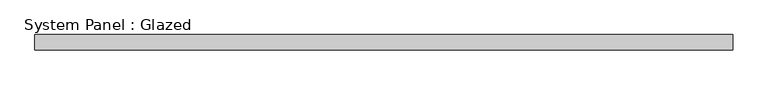
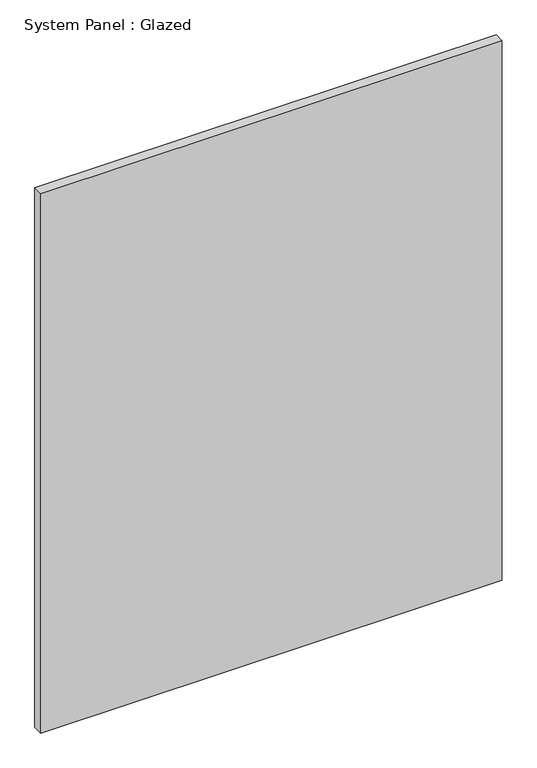
"""IFC4 building model written with IfcOpenShell, lengths in millimetres: plate geometry, System Panel : Glazed."""

import ifcopenshell
import ifcopenshell.guid

model = None  # the IFC model being written
_history = None  # IfcOwnerHistory: only IFC2X3 demands one
_inside = {}  # id of a spatial element -> (the spatial element, [elements in it])
_under = {}  # id of a project, library or spatial element -> (it, [spatial elements below it])
_declared = {}  # id of a project -> (the project, [libraries it declares])
_typed = {}  # id of a type object -> (the type object, [elements of that type])
_made_of = {}  # id of a material, layer set ... -> (it, [elements and type objects made of it])


def new_model(schema):
    """Start an empty IFC model of exactly this schema.

    Asked for "IFC4X3", IfcOpenShell would pick the latest addendum, in which some entities
    have other attributes; the version numbers below select the first issue.
    IFC2X3 requires an IfcOwnerHistory on every rooted entity: one is made here for all.
    """
    global model, _history
    if schema == "IFC4X3":
        model = ifcopenshell.file(schema_version=(4, 3, 0, 0))
    else:
        model = ifcopenshell.file(schema=schema)
    _inside.clear()
    _under.clear()
    _declared.clear()
    _typed.clear()
    _made_of.clear()
    _history = None
    if model.schema == "IFC2X3":
        org = make("IfcOrganization", Name="unknown")
        user = make(
            "IfcPersonAndOrganization",
            ThePerson=make("IfcPerson", FamilyName="unknown"),
            TheOrganization=org,
        )
        app = make(
            "IfcApplication",
            ApplicationDeveloper=org,
            Version="unknown",
            ApplicationFullName="unknown",
            ApplicationIdentifier="unknown",
        )
        _history = make(
            "IfcOwnerHistory",
            OwningUser=user,
            OwningApplication=app,
            ChangeAction="ADDED",
            CreationDate=0,
        )
    return model


def make(cls, **values):
    """One entity of the class cls with the attributes given. An attribute that is None is left unset."""
    return model.create_entity(
        cls, **{name: value for name, value in values.items() if value is not None}
    )


def rooted(cls, **values):
    """An entity with a GlobalId (a new one), such as an element, a storey or a relation."""
    return make(cls, GlobalId=ifcopenshell.guid.new(), OwnerHistory=_history, **values)


def si_unit(unit_type, name, prefix=None):
    """IfcSIUnit, for example si_unit("LENGTHUNIT", "METRE", prefix="MILLI")."""
    return make("IfcSIUnit", UnitType=unit_type, Prefix=prefix, Name=name)


def assignment(units):
    """IfcUnitAssignment: the units of a project."""
    return None if units is None else make("IfcUnitAssignment", Units=units)


def point(xyz):
    """IfcCartesianPoint."""
    return None if xyz is None else make("IfcCartesianPoint", Coordinates=xyz)


def direction(xyz):
    """IfcDirection."""
    return None if xyz is None else make("IfcDirection", DirectionRatios=xyz)


def frame(location, z_axis=None, x_axis=None):
    """IfcAxis2Placement3D, a coordinate frame: its origin and axes. An axis left out is left unset."""
    return make(
        "IfcAxis2Placement3D",
        Location=point(location),
        Axis=direction(z_axis),
        RefDirection=direction(x_axis),
    )


def origin():
    """The frame at (0, 0, 0) with its axes left unset."""
    return frame((0.0, 0.0, 0.0))


def origin_with_axes():
    """The frame at (0, 0, 0) with the z axis (0, 0, 1) and the x axis (1, 0, 0) written out."""
    return frame((0.0, 0.0, 0.0), z_axis=(0.0, 0.0, 1.0), x_axis=(1.0, 0.0, 0.0))


def place(relative_to, where):
    """IfcLocalPlacement: puts the frame where relative to a parent placement (None: the world)."""
    return make(
        "IfcLocalPlacement", PlacementRelTo=relative_to, RelativePlacement=where
    )


def context(
    kind, dimensions, precision=None, world=None, true_north=None, identifier=None
):
    """IfcGeometricRepresentationContext, for example the 3D "Model" context."""
    return make(
        "IfcGeometricRepresentationContext",
        ContextIdentifier=identifier,
        ContextType=kind,
        CoordinateSpaceDimension=dimensions,
        Precision=precision,
        WorldCoordinateSystem=world,
        TrueNorth=true_north,
    )


def project(units=None, contexts=None):
    """IfcProject with its units and contexts."""
    return rooted(
        "IfcProject",
        Name="project",
        RepresentationContexts=contexts,
        UnitsInContext=assignment(units),
    )


def spatial(cls, under=None, at=None, **own):
    """A site, building, storey or space (cls), placed at a placement, below another one or the project."""
    s = rooted(cls, ObjectPlacement=at, **own)
    if under is not None:
        _under.setdefault(under.id(), (under, []))[1].append(s)
    return s


def polyline(points):
    """IfcPolyline through the points."""
    return make("IfcPolyline", Points=[point(p) for p in points])


def outline(outer, holes=None, kind="AREA"):
    """IfcArbitraryClosedProfileDef: a profile drawn as a closed curve; with holes, ...WithVoids."""
    if holes is None:
        return make("IfcArbitraryClosedProfileDef", ProfileType=kind, OuterCurve=outer)
    return make(
        "IfcArbitraryProfileDefWithVoids",
        ProfileType=kind,
        OuterCurve=outer,
        InnerCurves=holes,
    )


def extrude(swept, where, along, depth):
    """IfcExtrudedAreaSolid: the profile swept, set in the frame where, extruded along a direction by depth."""
    return make(
        "IfcExtrudedAreaSolid",
        SweptArea=swept,
        Position=where,
        ExtrudedDirection=direction(along),
        Depth=depth,
    )


def shape(context_of_items, identifier, shape_type, items):
    """IfcShapeRepresentation: the items that make up one representation, for example the "Body"."""
    return make(
        "IfcShapeRepresentation",
        ContextOfItems=context_of_items,
        RepresentationIdentifier=identifier,
        RepresentationType=shape_type,
        Items=items,
    )


def source(mapping_origin, context_of_items, identifier, shape_type, items):
    """IfcRepresentationMap: a shape defined once, which mapped items show again and again."""
    return make(
        "IfcRepresentationMap",
        MappingOrigin=mapping_origin,
        MappedRepresentation=shape(context_of_items, identifier, shape_type, items),
    )


def transform(
    local_origin,
    x_axis=None,
    y_axis=None,
    z_axis=None,
    scale=None,
    scale2=None,
    scale3=None,
    uniform=True,
):
    """IfcCartesianTransformationOperator3D, or its non-uniform kind. x_axis, y_axis, z_axis: its Axis1, 2, 3."""
    if uniform:
        return make(
            "IfcCartesianTransformationOperator3D",
            Axis1=direction(x_axis),
            Axis2=direction(y_axis),
            LocalOrigin=point(local_origin),
            Scale=scale,
            Axis3=direction(z_axis),
        )
    return make(
        "IfcCartesianTransformationOperator3DnonUniform",
        Axis1=direction(x_axis),
        Axis2=direction(y_axis),
        LocalOrigin=point(local_origin),
        Scale=scale,
        Axis3=direction(z_axis),
        Scale2=scale2,
        Scale3=scale3,
    )


def mapped(mapping_source, mapping_target):
    """IfcMappedItem: shows the shape of a source again, moved by a transform."""
    return make(
        "IfcMappedItem", MappingSource=mapping_source, MappingTarget=mapping_target
    )


def made_of(thing, what):
    """Note that an element or type object is made of a material, layer set ...; save() writes the relation."""
    if what is not None:
        _made_of.setdefault(what.id(), (what, []))[1].append(thing)
    return thing


def element(
    cls,
    number,
    at=None,
    inside=None,
    cuts=None,
    type_object=None,
    material=None,
    context=None,
    identifier="Body",
    shape_type=None,
    held_by="IfcProductDefinitionShape",
    body=None,
    shapes=None,
    **own,
):
    """One element of the class cls, such as IfcWall. Its Tag is "e" and its number.

    at: its placement. inside: the storey or other place that contains it. cuts: it is an
    opening in that element (IfcRelVoidsElement). A single representation is given by context,
    identifier, shape_type and body (its items); several are given by shapes. held_by: the class
    of the entity that holds the representations. save() writes the other relations.
    """
    e = rooted(cls, Tag="e%d" % number, ObjectPlacement=at, **own)
    if body is not None:
        shapes = [shape(context, identifier, shape_type, body)]
    if shapes is not None:
        e.Representation = make(held_by, Representations=shapes)
    if inside is not None:
        _inside.setdefault(inside.id(), (inside, []))[1].append(e)
    if cuts is not None:
        rooted(
            "IfcRelVoidsElement", RelatingBuildingElement=cuts, RelatedOpeningElement=e
        )
    if type_object is not None:
        _typed.setdefault(type_object.id(), (type_object, []))[1].append(e)
    return made_of(e, material)


def aggregate(whole, parts):
    """IfcRelAggregates: a whole, such as a stair, and the parts it consists of."""
    return rooted("IfcRelAggregates", RelatingObject=whole, RelatedObjects=parts)


def save(model, path):
    """Write the relations noted so far, then the file.

    IfcRelAggregates (storeys below a building ...), IfcRelContainedInSpatialStructure (elements
    in a storey), IfcRelDefinesByType, IfcRelAssociatesMaterial and IfcRelDeclares: one each for
    every whole, place, type object, material and project.
    """
    for whole, parts in _under.values():
        aggregate(whole, parts)
    for where, things in _inside.values():
        rooted(
            "IfcRelContainedInSpatialStructure",
            RelatedElements=things,
            RelatingStructure=where,
        )
    for kind, things in _typed.values():
        rooted("IfcRelDefinesByType", RelatedObjects=things, RelatingType=kind)
    for what, things in _made_of.values():
        rooted("IfcRelAssociatesMaterial", RelatedObjects=things, RelatingMaterial=what)
    for by, libraries in _declared.values():
        rooted("IfcRelDeclares", RelatingContext=by, RelatedDefinitions=libraries)
    model.write(path)


def system_panel_glazed_b81d08ea(model_context):
    return source(origin(), model_context, "Body", "SweptSolid", [
        extrude(outline(polyline([(566.6666667, 24.5), (-566.6666667, 24.5), (-566.6666667, 49.5), (566.6666667, 49.5), (566.6666667, 24.5)])), origin_with_axes(), (0.0, 0.0, 1.0), 1400.0),
    ])


if __name__ == "__main__":
    model = new_model("IFC4")
    model_context = context("Model", 3, world=origin())
    ifc_project = project(units=[si_unit("LENGTHUNIT", "METRE", prefix="MILLI")], contexts=[model_context])
    site = spatial("IfcSite", under=ifc_project)
    building = spatial("IfcBuilding", under=site)
    placement = place(None, origin())
    system_panel_glazed_shape = system_panel_glazed_b81d08ea(model_context)
    element("IfcPlate", 1, ObjectType="System Panel : Glazed", at=placement, inside=building, context=model_context, shape_type="MappedRepresentation", body=[
        mapped(system_panel_glazed_shape, transform((0.0, 0.0, 0.0), x_axis=(1.0, 0.0, 0.0), y_axis=(0.0, 1.0, 0.0), z_axis=(0.0, 0.0, 1.0))),
    ])
    save(model, "model.ifc")

# Revit data of these elements
# Element 1 (IfcPlate, "System Panel : Glazed")
#   Materials on its faces: "Glass"
# Materials
#   "Glass": class "Glass", colour RGB 0 128 192, transparency 0.9
